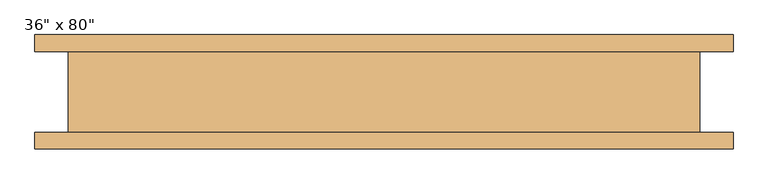
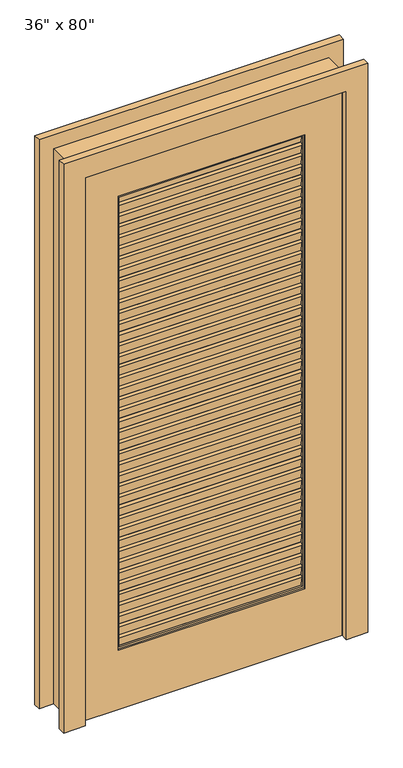
"""IFC4 building model written with IfcOpenShell, lengths in millimetres: door geometry."""

import ifcopenshell
import ifcopenshell.guid

model = None  # the IFC model being written
_history = None  # IfcOwnerHistory: only IFC2X3 demands one
_inside = {}  # id of a spatial element -> (the spatial element, [elements in it])
_under = {}  # id of a project, library or spatial element -> (it, [spatial elements below it])
_declared = {}  # id of a project -> (the project, [libraries it declares])
_typed = {}  # id of a type object -> (the type object, [elements of that type])
_made_of = {}  # id of a material, layer set ... -> (it, [elements and type objects made of it])


def new_model(schema):
    """Start an empty IFC model of exactly this schema.

    Asked for "IFC4X3", IfcOpenShell would pick the latest addendum, in which some entities
    have other attributes; the version numbers below select the first issue.
    IFC2X3 requires an IfcOwnerHistory on every rooted entity: one is made here for all.
    """
    global model, _history
    if schema == "IFC4X3":
        model = ifcopenshell.file(schema_version=(4, 3, 0, 0))
    else:
        model = ifcopenshell.file(schema=schema)
    _inside.clear()
    _under.clear()
    _declared.clear()
    _typed.clear()
    _made_of.clear()
    _history = None
    if model.schema == "IFC2X3":
        org = make("IfcOrganization", Name="unknown")
        user = make(
            "IfcPersonAndOrganization",
            ThePerson=make("IfcPerson", FamilyName="unknown"),
            TheOrganization=org,
        )
        app = make(
            "IfcApplication",
            ApplicationDeveloper=org,
            Version="unknown",
            ApplicationFullName="unknown",
            ApplicationIdentifier="unknown",
        )
        _history = make(
            "IfcOwnerHistory",
            OwningUser=user,
            OwningApplication=app,
            ChangeAction="ADDED",
            CreationDate=0,
        )
    return model


def make(cls, **values):
    """One entity of the class cls with the attributes given. An attribute that is None is left unset."""
    return model.create_entity(
        cls, **{name: value for name, value in values.items() if value is not None}
    )


def rooted(cls, **values):
    """An entity with a GlobalId (a new one), such as an element, a storey or a relation."""
    return make(cls, GlobalId=ifcopenshell.guid.new(), OwnerHistory=_history, **values)


def si_unit(unit_type, name, prefix=None):
    """IfcSIUnit, for example si_unit("LENGTHUNIT", "METRE", prefix="MILLI")."""
    return make("IfcSIUnit", UnitType=unit_type, Prefix=prefix, Name=name)


def assignment(units):
    """IfcUnitAssignment: the units of a project."""
    return None if units is None else make("IfcUnitAssignment", Units=units)


def point(xyz):
    """IfcCartesianPoint."""
    return None if xyz is None else make("IfcCartesianPoint", Coordinates=xyz)


def direction(xyz):
    """IfcDirection."""
    return None if xyz is None else make("IfcDirection", DirectionRatios=xyz)


def frame(location, z_axis=None, x_axis=None):
    """IfcAxis2Placement3D, a coordinate frame: its origin and axes. An axis left out is left unset."""
    return make(
        "IfcAxis2Placement3D",
        Location=point(location),
        Axis=direction(z_axis),
        RefDirection=direction(x_axis),
    )


def frame_2d(location, x_axis=None):
    """IfcAxis2Placement2D, a coordinate frame in the plane: its origin and x axis."""
    return make(
        "IfcAxis2Placement2D", Location=point(location), RefDirection=direction(x_axis)
    )


def origin():
    """The frame at (0, 0, 0) with its axes left unset."""
    return frame((0.0, 0.0, 0.0))


def place(relative_to, where):
    """IfcLocalPlacement: puts the frame where relative to a parent placement (None: the world)."""
    return make(
        "IfcLocalPlacement", PlacementRelTo=relative_to, RelativePlacement=where
    )


def context(
    kind, dimensions, precision=None, world=None, true_north=None, identifier=None
):
    """IfcGeometricRepresentationContext, for example the 3D "Model" context."""
    return make(
        "IfcGeometricRepresentationContext",
        ContextIdentifier=identifier,
        ContextType=kind,
        CoordinateSpaceDimension=dimensions,
        Precision=precision,
        WorldCoordinateSystem=world,
        TrueNorth=true_north,
    )


def project(units=None, contexts=None):
    """IfcProject with its units and contexts."""
    return rooted(
        "IfcProject",
        Name="project",
        RepresentationContexts=contexts,
        UnitsInContext=assignment(units),
    )


def spatial(cls, under=None, at=None, **own):
    """A site, building, storey or space (cls), placed at a placement, below another one or the project."""
    s = rooted(cls, ObjectPlacement=at, **own)
    if under is not None:
        _under.setdefault(under.id(), (under, []))[1].append(s)
    return s


def polyline(points):
    """IfcPolyline through the points."""
    return make("IfcPolyline", Points=[point(p) for p in points])


def circle_curve(where, radius):
    """IfcCircle in the frame where."""
    return make("IfcCircle", Position=where, Radius=radius)


def trimmed(basis, trim1, trim2, sense, master):
    """IfcTrimmedCurve: the piece of a basis curve between two trims."""
    return make(
        "IfcTrimmedCurve",
        BasisCurve=basis,
        Trim1=trim1,
        Trim2=trim2,
        SenseAgreement=sense,
        MasterRepresentation=master,
    )


def segment(curve, same_sense, transition):
    """IfcCompositeCurveSegment."""
    return make(
        "IfcCompositeCurveSegment",
        Transition=transition,
        SameSense=same_sense,
        ParentCurve=curve,
    )


def composite_curve(segments, self_intersect=None):
    """IfcCompositeCurve: segments joined end to end."""
    return make("IfcCompositeCurve", Segments=segments, SelfIntersect=self_intersect)


def outline(outer, holes=None, kind="AREA"):
    """IfcArbitraryClosedProfileDef: a profile drawn as a closed curve; with holes, ...WithVoids."""
    if holes is None:
        return make("IfcArbitraryClosedProfileDef", ProfileType=kind, OuterCurve=outer)
    return make(
        "IfcArbitraryProfileDefWithVoids",
        ProfileType=kind,
        OuterCurve=outer,
        InnerCurves=holes,
    )


def extrude(swept, where, along, depth):
    """IfcExtrudedAreaSolid: the profile swept, set in the frame where, extruded along a direction by depth."""
    return make(
        "IfcExtrudedAreaSolid",
        SweptArea=swept,
        Position=where,
        ExtrudedDirection=direction(along),
        Depth=depth,
    )


def faces_of(points, faces, orient=None, outer=None):
    """IfcFace entities. A face is a list of loops; a loop is a list of indices into points, from 0.

    orient and outer hold one flag for each loop. By default every Orientation is true, the
    first loop of a face is its IfcFaceOuterBound and the others are IfcFaceBound.
    """
    made = []
    for i, loops in enumerate(faces):
        bounds = []
        for j, loop in enumerate(loops):
            is_outer = j == 0 if outer is None else outer[i][j]
            bounds.append(
                make(
                    "IfcFaceOuterBound" if is_outer else "IfcFaceBound",
                    Bound=make("IfcPolyLoop", Polygon=[points[k] for k in loop]),
                    Orientation=True if orient is None else orient[i][j],
                )
            )
        made.append(make("IfcFace", Bounds=bounds))
    return made


def faceted_brep(points, faces, orient=None, outer=None, voids=None):
    """IfcFacetedBrep: a solid bounded by flat faces; with voids (closed shells), ...WithVoids."""
    shared = [point(p) for p in points]
    hull = make("IfcClosedShell", CfsFaces=faces_of(shared, faces, orient, outer))
    if voids is None:
        return make("IfcFacetedBrep", Outer=hull)
    return make(
        "IfcFacetedBrepWithVoids",
        Outer=hull,
        Voids=[
            make(cls, CfsFaces=faces_of(shared, fs, o, b)) for cls, fs, o, b in voids
        ],
    )


def shape(context_of_items, identifier, shape_type, items):
    """IfcShapeRepresentation: the items that make up one representation, for example the "Body"."""
    return make(
        "IfcShapeRepresentation",
        ContextOfItems=context_of_items,
        RepresentationIdentifier=identifier,
        RepresentationType=shape_type,
        Items=items,
    )


def source(mapping_origin, context_of_items, identifier, shape_type, items):
    """IfcRepresentationMap: a shape defined once, which mapped items show again and again."""
    return make(
        "IfcRepresentationMap",
        MappingOrigin=mapping_origin,
        MappedRepresentation=shape(context_of_items, identifier, shape_type, items),
    )


def transform(
    local_origin,
    x_axis=None,
    y_axis=None,
    z_axis=None,
    scale=None,
    scale2=None,
    scale3=None,
    uniform=True,
):
    """IfcCartesianTransformationOperator3D, or its non-uniform kind. x_axis, y_axis, z_axis: its Axis1, 2, 3."""
    if uniform:
        return make(
            "IfcCartesianTransformationOperator3D",
            Axis1=direction(x_axis),
            Axis2=direction(y_axis),
            LocalOrigin=point(local_origin),
            Scale=scale,
            Axis3=direction(z_axis),
        )
    return make(
        "IfcCartesianTransformationOperator3DnonUniform",
        Axis1=direction(x_axis),
        Axis2=direction(y_axis),
        LocalOrigin=point(local_origin),
        Scale=scale,
        Axis3=direction(z_axis),
        Scale2=scale2,
        Scale3=scale3,
    )


def mapped(mapping_source, mapping_target):
    """IfcMappedItem: shows the shape of a source again, moved by a transform."""
    return make(
        "IfcMappedItem", MappingSource=mapping_source, MappingTarget=mapping_target
    )


def made_of(thing, what):
    """Note that an element or type object is made of a material, layer set ...; save() writes the relation."""
    if what is not None:
        _made_of.setdefault(what.id(), (what, []))[1].append(thing)
    return thing


def element(
    cls,
    number,
    at=None,
    inside=None,
    cuts=None,
    type_object=None,
    material=None,
    context=None,
    identifier="Body",
    shape_type=None,
    held_by="IfcProductDefinitionShape",
    body=None,
    shapes=None,
    **own,
):
    """One element of the class cls, such as IfcWall. Its Tag is "e" and its number.

    at: its placement. inside: the storey or other place that contains it. cuts: it is an
    opening in that element (IfcRelVoidsElement). A single representation is given by context,
    identifier, shape_type and body (its items); several are given by shapes. held_by: the class
    of the entity that holds the representations. save() writes the other relations.
    """
    e = rooted(cls, Tag="e%d" % number, ObjectPlacement=at, **own)
    if body is not None:
        shapes = [shape(context, identifier, shape_type, body)]
    if shapes is not None:
        e.Representation = make(held_by, Representations=shapes)
    if inside is not None:
        _inside.setdefault(inside.id(), (inside, []))[1].append(e)
    if cuts is not None:
        rooted(
            "IfcRelVoidsElement", RelatingBuildingElement=cuts, RelatedOpeningElement=e
        )
    if type_object is not None:
        _typed.setdefault(type_object.id(), (type_object, []))[1].append(e)
    return made_of(e, material)


def aggregate(whole, parts):
    """IfcRelAggregates: a whole, such as a stair, and the parts it consists of."""
    return rooted("IfcRelAggregates", RelatingObject=whole, RelatedObjects=parts)


def save(model, path):
    """Write the relations noted so far, then the file.

    IfcRelAggregates (storeys below a building ...), IfcRelContainedInSpatialStructure (elements
    in a storey), IfcRelDefinesByType, IfcRelAssociatesMaterial and IfcRelDeclares: one each for
    every whole, place, type object, material and project.
    """
    for whole, parts in _under.values():
        aggregate(whole, parts)
    for where, things in _inside.values():
        rooted(
            "IfcRelContainedInSpatialStructure",
            RelatedElements=things,
            RelatingStructure=where,
        )
    for kind, things in _typed.values():
        rooted("IfcRelDefinesByType", RelatedObjects=things, RelatingType=kind)
    for what, things in _made_of.values():
        rooted("IfcRelAssociatesMaterial", RelatedObjects=things, RelatingMaterial=what)
    for by, libraries in _declared.values():
        rooted("IfcRelDeclares", RelatingContext=by, RelatedDefinitions=libraries)
    model.write(path)


def door_294ae2c4(model_context):
    return source(origin(), model_context, "Body", "SolidModel", [
        extrude(outline(composite_curve([segment(polyline([(-25.516257, 1899.8217262), (-31.75, 1867.3157738), (-31.75, 1857.7907738), (-47.625, 1857.7907738), (-47.625, 1867.3157738), (-53.858743, 1899.8217262)]), True, "CONTINUOUS"), segment(trimmed(circle_curve(frame_2d((-47.625, 1901.03125)), 6.35), [point((-53.858743, 1899.8217262))], [point((-47.625, 1907.38125))], False, "CARTESIAN"), True, "CONTINUOUS"), segment(polyline([(-47.625, 1907.38125), (-47.625, 1899.44375), (-31.75, 1899.44375), (-31.75, 1907.38125)]), True, "CONTINUOUS"), segment(trimmed(circle_curve(frame_2d((-31.75, 1901.03125)), 6.35), [point((-31.75, 1907.38125))], [point((-25.516257, 1899.8217262))], False, "CARTESIAN"), True, "CONTINUOUS")], self_intersect=False)), frame((-327.025, 0.0, 0.0), z_axis=(1.0, 0.0, 0.0), x_axis=(0.0, 1.0, 0.0)), (0.0, 0.0, 1.0), 654.05),
        extrude(outline(composite_curve([segment(polyline([(-25.516257, 1859.75625), (-31.75, 1827.2502976), (-31.75, 1817.7252976), (-47.625, 1817.7252976), (-47.625, 1827.2502976), (-53.858743, 1859.75625)]), True, "CONTINUOUS"), segment(trimmed(circle_curve(frame_2d((-47.625, 1860.9657738)), 6.35), [point((-53.858743, 1859.75625))], [point((-47.625, 1867.3157738))], False, "CARTESIAN"), True, "CONTINUOUS"), segment(polyline([(-47.625, 1867.3157738), (-47.625, 1859.3782738), (-31.75, 1859.3782738), (-31.75, 1867.3157738)]), True, "CONTINUOUS"), segment(trimmed(circle_curve(frame_2d((-31.75, 1860.9657738)), 6.35), [point((-31.75, 1867.3157738))], [point((-25.516257, 1859.75625))], False, "CARTESIAN"), True, "CONTINUOUS")], self_intersect=False)), frame((-327.025, 0.0, 0.0), z_axis=(1.0, 0.0, 0.0), x_axis=(0.0, 1.0, 0.0)), (0.0, 0.0, 1.0), 654.05),
        extrude(outline(composite_curve([segment(polyline([(-25.516257, 1819.6907738), (-31.75, 1787.1848214), (-31.75, 1777.6598214), (-47.625, 1777.6598214), (-47.625, 1787.1848214), (-53.858743, 1819.6907738)]), True, "CONTINUOUS"), segment(trimmed(circle_curve(frame_2d((-47.625, 1820.9002976)), 6.35), [point((-53.858743, 1819.6907738))], [point((-47.625, 1827.2502976))], False, "CARTESIAN"), True, "CONTINUOUS"), segment(polyline([(-47.625, 1827.2502976), (-47.625, 1819.3127976), (-31.75, 1819.3127976), (-31.75, 1827.2502976)]), True, "CONTINUOUS"), segment(trimmed(circle_curve(frame_2d((-31.75, 1820.9002976)), 6.35), [point((-31.75, 1827.2502976))], [point((-25.516257, 1819.6907738))], False, "CARTESIAN"), True, "CONTINUOUS")], self_intersect=False)), frame((-327.025, 0.0, 0.0), z_axis=(1.0, 0.0, 0.0), x_axis=(0.0, 1.0, 0.0)), (0.0, 0.0, 1.0), 654.05),
        extrude(outline(composite_curve([segment(polyline([(-25.516257, 1779.6252976), (-31.75, 1747.1193452), (-31.75, 1737.5943452), (-47.625, 1737.5943452), (-47.625, 1747.1193452), (-53.858743, 1779.6252976)]), True, "CONTINUOUS"), segment(trimmed(circle_curve(frame_2d((-47.625, 1780.8348214)), 6.35), [point((-53.858743, 1779.6252976))], [point((-47.625, 1787.1848214))], False, "CARTESIAN"), True, "CONTINUOUS"), segment(polyline([(-47.625, 1787.1848214), (-47.625, 1779.2473214), (-31.75, 1779.2473214), (-31.75, 1787.1848214)]), True, "CONTINUOUS"), segment(trimmed(circle_curve(frame_2d((-31.75, 1780.8348214)), 6.35), [point((-31.75, 1787.1848214))], [point((-25.516257, 1779.6252976))], False, "CARTESIAN"), True, "CONTINUOUS")], self_intersect=False)), frame((-327.025, 0.0, 0.0), z_axis=(1.0, 0.0, 0.0), x_axis=(0.0, 1.0, 0.0)), (0.0, 0.0, 1.0), 654.05),
        extrude(outline(composite_curve([segment(polyline([(-25.516257, 1739.5598214), (-31.75, 1707.053869), (-31.75, 1697.528869), (-47.625, 1697.528869), (-47.625, 1707.053869), (-53.858743, 1739.5598214)]), True, "CONTINUOUS"), segment(trimmed(circle_curve(frame_2d((-47.625, 1740.7693452)), 6.35), [point((-53.858743, 1739.5598214))], [point((-47.625, 1747.1193452))], False, "CARTESIAN"), True, "CONTINUOUS"), segment(polyline([(-47.625, 1747.1193452), (-47.625, 1739.1818452), (-31.75, 1739.1818452), (-31.75, 1747.1193452)]), True, "CONTINUOUS"), segment(trimmed(circle_curve(frame_2d((-31.75, 1740.7693452)), 6.35), [point((-31.75, 1747.1193452))], [point((-25.516257, 1739.5598214))], False, "CARTESIAN"), True, "CONTINUOUS")], self_intersect=False)), frame((-327.025, 0.0, 0.0), z_axis=(1.0, 0.0, 0.0), x_axis=(0.0, 1.0, 0.0)), (0.0, 0.0, 1.0), 654.05),
        extrude(outline(composite_curve([segment(polyline([(-25.516257, 1699.4943452), (-31.75, 1666.9883929), (-31.75, 1657.4633929), (-47.625, 1657.4633929), (-47.625, 1666.9883929), (-53.858743, 1699.4943452)]), True, "CONTINUOUS"), segment(trimmed(circle_curve(frame_2d((-47.625, 1700.703869)), 6.35), [point((-53.858743, 1699.4943452))], [point((-47.625, 1707.053869))], False, "CARTESIAN"), True, "CONTINUOUS"), segment(polyline([(-47.625, 1707.053869), (-47.625, 1699.116369), (-31.75, 1699.116369), (-31.75, 1707.053869)]), True, "CONTINUOUS"), segment(trimmed(circle_curve(frame_2d((-31.75, 1700.703869)), 6.35), [point((-31.75, 1707.053869))], [point((-25.516257, 1699.4943452))], False, "CARTESIAN"), True, "CONTINUOUS")], self_intersect=False)), frame((-327.025, 0.0, 0.0), z_axis=(1.0, 0.0, 0.0), x_axis=(0.0, 1.0, 0.0)), (0.0, 0.0, 1.0), 654.05),
        extrude(outline(composite_curve([segment(polyline([(-25.516257, 1659.428869), (-31.75, 1626.9229167), (-31.75, 1617.3979167), (-47.625, 1617.3979167), (-47.625, 1626.9229167), (-53.858743, 1659.428869)]), True, "CONTINUOUS"), segment(trimmed(circle_curve(frame_2d((-47.625, 1660.6383929)), 6.35), [point((-53.858743, 1659.428869))], [point((-47.625, 1666.9883929))], False, "CARTESIAN"), True, "CONTINUOUS"), segment(polyline([(-47.625, 1666.9883929), (-47.625, 1659.0508929), (-31.75, 1659.0508929), (-31.75, 1666.9883929)]), True, "CONTINUOUS"), segment(trimmed(circle_curve(frame_2d((-31.75, 1660.6383929)), 6.35), [point((-31.75, 1666.9883929))], [point((-25.516257, 1659.428869))], False, "CARTESIAN"), True, "CONTINUOUS")], self_intersect=False)), frame((-327.025, 0.0, 0.0), z_axis=(1.0, 0.0, 0.0), x_axis=(0.0, 1.0, 0.0)), (0.0, 0.0, 1.0), 654.05),
        extrude(outline(composite_curve([segment(polyline([(-25.516257, 1619.3633929), (-31.75, 1586.8574405), (-31.75, 1577.3324405), (-47.625, 1577.3324405), (-47.625, 1586.8574405), (-53.858743, 1619.3633929)]), True, "CONTINUOUS"), segment(trimmed(circle_curve(frame_2d((-47.625, 1620.5729167)), 6.35), [point((-53.858743, 1619.3633929))], [point((-47.625, 1626.9229167))], False, "CARTESIAN"), True, "CONTINUOUS"), segment(polyline([(-47.625, 1626.9229167), (-47.625, 1618.9854167), (-31.75, 1618.9854167), (-31.75, 1626.9229167)]), True, "CONTINUOUS"), segment(trimmed(circle_curve(frame_2d((-31.75, 1620.5729167)), 6.35), [point((-31.75, 1626.9229167))], [point((-25.516257, 1619.3633929))], False, "CARTESIAN"), True, "CONTINUOUS")], self_intersect=False)), frame((-327.025, 0.0, 0.0), z_axis=(1.0, 0.0, 0.0), x_axis=(0.0, 1.0, 0.0)), (0.0, 0.0, 1.0), 654.05),
        extrude(outline(composite_curve([segment(polyline([(-25.516257, 1579.2979167), (-31.75, 1546.7919643), (-31.75, 1537.2669643), (-47.625, 1537.2669643), (-47.625, 1546.7919643), (-53.858743, 1579.2979167)]), True, "CONTINUOUS"), segment(trimmed(circle_curve(frame_2d((-47.625, 1580.5074405)), 6.35), [point((-53.858743, 1579.2979167))], [point((-47.625, 1586.8574405))], False, "CARTESIAN"), True, "CONTINUOUS"), segment(polyline([(-47.625, 1586.8574405), (-47.625, 1578.9199405), (-31.75, 1578.9199405), (-31.75, 1586.8574405)]), True, "CONTINUOUS"), segment(trimmed(circle_curve(frame_2d((-31.75, 1580.5074405)), 6.35), [point((-31.75, 1586.8574405))], [point((-25.516257, 1579.2979167))], False, "CARTESIAN"), True, "CONTINUOUS")], self_intersect=False)), frame((-327.025, 0.0, 0.0), z_axis=(1.0, 0.0, 0.0), x_axis=(0.0, 1.0, 0.0)), (0.0, 0.0, 1.0), 654.05),
        extrude(outline(composite_curve([segment(polyline([(-25.516257, 1539.2324405), (-31.75, 1506.7264881), (-31.75, 1497.2014881), (-47.625, 1497.2014881), (-47.625, 1506.7264881), (-53.858743, 1539.2324405)]), True, "CONTINUOUS"), segment(trimmed(circle_curve(frame_2d((-47.625, 1540.4419643)), 6.35), [point((-53.858743, 1539.2324405))], [point((-47.625, 1546.7919643))], False, "CARTESIAN"), True, "CONTINUOUS"), segment(polyline([(-47.625, 1546.7919643), (-47.625, 1538.8544643), (-31.75, 1538.8544643), (-31.75, 1546.7919643)]), True, "CONTINUOUS"), segment(trimmed(circle_curve(frame_2d((-31.75, 1540.4419643)), 6.35), [point((-31.75, 1546.7919643))], [point((-25.516257, 1539.2324405))], False, "CARTESIAN"), True, "CONTINUOUS")], self_intersect=False)), frame((-327.025, 0.0, 0.0), z_axis=(1.0, 0.0, 0.0), x_axis=(0.0, 1.0, 0.0)), (0.0, 0.0, 1.0), 654.05),
        extrude(outline(composite_curve([segment(polyline([(-25.516257, 1499.1669643), (-31.75, 1466.6610119), (-31.75, 1457.1360119), (-47.625, 1457.1360119), (-47.625, 1466.6610119), (-53.858743, 1499.1669643)]), True, "CONTINUOUS"), segment(trimmed(circle_curve(frame_2d((-47.625, 1500.3764881)), 6.35), [point((-53.858743, 1499.1669643))], [point((-47.625, 1506.7264881))], False, "CARTESIAN"), True, "CONTINUOUS"), segment(polyline([(-47.625, 1506.7264881), (-47.625, 1498.7889881), (-31.75, 1498.7889881), (-31.75, 1506.7264881)]), True, "CONTINUOUS"), segment(trimmed(circle_curve(frame_2d((-31.75, 1500.3764881)), 6.35), [point((-31.75, 1506.7264881))], [point((-25.516257, 1499.1669643))], False, "CARTESIAN"), True, "CONTINUOUS")], self_intersect=False)), frame((-327.025, 0.0, 0.0), z_axis=(1.0, 0.0, 0.0), x_axis=(0.0, 1.0, 0.0)), (0.0, 0.0, 1.0), 654.05),
        extrude(outline(composite_curve([segment(polyline([(-25.516257, 1459.1014881), (-31.75, 1426.5955357), (-31.75, 1417.0705357), (-47.625, 1417.0705357), (-47.625, 1426.5955357), (-53.858743, 1459.1014881)]), True, "CONTINUOUS"), segment(trimmed(circle_curve(frame_2d((-47.625, 1460.3110119)), 6.35), [point((-53.858743, 1459.1014881))], [point((-47.625, 1466.6610119))], False, "CARTESIAN"), True, "CONTINUOUS"), segment(polyline([(-47.625, 1466.6610119), (-47.625, 1458.7235119), (-31.75, 1458.7235119), (-31.75, 1466.6610119)]), True, "CONTINUOUS"), segment(trimmed(circle_curve(frame_2d((-31.75, 1460.3110119)), 6.35), [point((-31.75, 1466.6610119))], [point((-25.516257, 1459.1014881))], False, "CARTESIAN"), True, "CONTINUOUS")], self_intersect=False)), frame((-327.025, 0.0, 0.0), z_axis=(1.0, 0.0, 0.0), x_axis=(0.0, 1.0, 0.0)), (0.0, 0.0, 1.0), 654.05),
        extrude(outline(composite_curve([segment(polyline([(-25.516257, 1419.0360119), (-31.75, 1386.5300595), (-31.75, 1377.0050595), (-47.625, 1377.0050595), (-47.625, 1386.5300595), (-53.858743, 1419.0360119)]), True, "CONTINUOUS"), segment(trimmed(circle_curve(frame_2d((-47.625, 1420.2455357)), 6.35), [point((-53.858743, 1419.0360119))], [point((-47.625, 1426.5955357))], False, "CARTESIAN"), True, "CONTINUOUS"), segment(polyline([(-47.625, 1426.5955357), (-47.625, 1418.6580357), (-31.75, 1418.6580357), (-31.75, 1426.5955357)]), True, "CONTINUOUS"), segment(trimmed(circle_curve(frame_2d((-31.75, 1420.2455357)), 6.35), [point((-31.75, 1426.5955357))], [point((-25.516257, 1419.0360119))], False, "CARTESIAN"), True, "CONTINUOUS")], self_intersect=False)), frame((-327.025, 0.0, 0.0), z_axis=(1.0, 0.0, 0.0), x_axis=(0.0, 1.0, 0.0)), (0.0, 0.0, 1.0), 654.05),
        extrude(outline(composite_curve([segment(polyline([(-25.516257, 1378.9705357), (-31.75, 1346.4645833), (-31.75, 1336.9395833), (-47.625, 1336.9395833), (-47.625, 1346.4645833), (-53.858743, 1378.9705357)]), True, "CONTINUOUS"), segment(trimmed(circle_curve(frame_2d((-47.625, 1380.1800595)), 6.35), [point((-53.858743, 1378.9705357))], [point((-47.625, 1386.5300595))], False, "CARTESIAN"), True, "CONTINUOUS"), segment(polyline([(-47.625, 1386.5300595), (-47.625, 1378.5925595), (-31.75, 1378.5925595), (-31.75, 1386.5300595)]), True, "CONTINUOUS"), segment(trimmed(circle_curve(frame_2d((-31.75, 1380.1800595)), 6.35), [point((-31.75, 1386.5300595))], [point((-25.516257, 1378.9705357))], False, "CARTESIAN"), True, "CONTINUOUS")], self_intersect=False)), frame((-327.025, 0.0, 0.0), z_axis=(1.0, 0.0, 0.0), x_axis=(0.0, 1.0, 0.0)), (0.0, 0.0, 1.0), 654.05),
        extrude(outline(composite_curve([segment(polyline([(-25.516257, 1338.9050595), (-31.75, 1306.3991071), (-31.75, 1296.8741071), (-47.625, 1296.8741071), (-47.625, 1306.3991071), (-53.858743, 1338.9050595)]), True, "CONTINUOUS"), segment(trimmed(circle_curve(frame_2d((-47.625, 1340.1145833)), 6.35), [point((-53.858743, 1338.9050595))], [point((-47.625, 1346.4645833))], False, "CARTESIAN"), True, "CONTINUOUS"), segment(polyline([(-47.625, 1346.4645833), (-47.625, 1338.5270833), (-31.75, 1338.5270833), (-31.75, 1346.4645833)]), True, "CONTINUOUS"), segment(trimmed(circle_curve(frame_2d((-31.75, 1340.1145833)), 6.35), [point((-31.75, 1346.4645833))], [point((-25.516257, 1338.9050595))], False, "CARTESIAN"), True, "CONTINUOUS")], self_intersect=False)), frame((-327.025, 0.0, 0.0), z_axis=(1.0, 0.0, 0.0), x_axis=(0.0, 1.0, 0.0)), (0.0, 0.0, 1.0), 654.05),
        extrude(outline(composite_curve([segment(polyline([(-25.516257, 1298.8395833), (-31.75, 1266.333631), (-31.75, 1256.808631), (-47.625, 1256.808631), (-47.625, 1266.333631), (-53.858743, 1298.8395833)]), True, "CONTINUOUS"), segment(trimmed(circle_curve(frame_2d((-47.625, 1300.0491071)), 6.35), [point((-53.858743, 1298.8395833))], [point((-47.625, 1306.3991071))], False, "CARTESIAN"), True, "CONTINUOUS"), segment(polyline([(-47.625, 1306.3991071), (-47.625, 1298.4616071), (-31.75, 1298.4616071), (-31.75, 1306.3991071)]), True, "CONTINUOUS"), segment(trimmed(circle_curve(frame_2d((-31.75, 1300.0491071)), 6.35), [point((-31.75, 1306.3991071))], [point((-25.516257, 1298.8395833))], False, "CARTESIAN"), True, "CONTINUOUS")], self_intersect=False)), frame((-327.025, 0.0, 0.0), z_axis=(1.0, 0.0, 0.0), x_axis=(0.0, 1.0, 0.0)), (0.0, 0.0, 1.0), 654.05),
        extrude(outline(composite_curve([segment(polyline([(-25.516257, 1258.7741071), (-31.75, 1226.2681548), (-31.75, 1216.7431548), (-47.625, 1216.7431548), (-47.625, 1226.2681548), (-53.858743, 1258.7741071)]), True, "CONTINUOUS"), segment(trimmed(circle_curve(frame_2d((-47.625, 1259.983631)), 6.35), [point((-53.858743, 1258.7741071))], [point((-47.625, 1266.333631))], False, "CARTESIAN"), True, "CONTINUOUS"), segment(polyline([(-47.625, 1266.333631), (-47.625, 1258.396131), (-31.75, 1258.396131), (-31.75, 1266.333631)]), True, "CONTINUOUS"), segment(trimmed(circle_curve(frame_2d((-31.75, 1259.983631)), 6.35), [point((-31.75, 1266.333631))], [point((-25.516257, 1258.7741071))], False, "CARTESIAN"), True, "CONTINUOUS")], self_intersect=False)), frame((-327.025, 0.0, 0.0), z_axis=(1.0, 0.0, 0.0), x_axis=(0.0, 1.0, 0.0)), (0.0, 0.0, 1.0), 654.05),
        extrude(outline(composite_curve([segment(polyline([(-25.516257, 1218.708631), (-31.75, 1186.2026786), (-31.75, 1176.6776786), (-47.625, 1176.6776786), (-47.625, 1186.2026786), (-53.858743, 1218.708631)]), True, "CONTINUOUS"), segment(trimmed(circle_curve(frame_2d((-47.625, 1219.9181548)), 6.35), [point((-53.858743, 1218.708631))], [point((-47.625, 1226.2681548))], False, "CARTESIAN"), True, "CONTINUOUS"), segment(polyline([(-47.625, 1226.2681548), (-47.625, 1218.3306548), (-31.75, 1218.3306548), (-31.75, 1226.2681548)]), True, "CONTINUOUS"), segment(trimmed(circle_curve(frame_2d((-31.75, 1219.9181548)), 6.35), [point((-31.75, 1226.2681548))], [point((-25.516257, 1218.708631))], False, "CARTESIAN"), True, "CONTINUOUS")], self_intersect=False)), frame((-327.025, 0.0, 0.0), z_axis=(1.0, 0.0, 0.0), x_axis=(0.0, 1.0, 0.0)), (0.0, 0.0, 1.0), 654.05),
        extrude(outline(composite_curve([segment(polyline([(-25.516257, 1178.6431548), (-31.75, 1146.1372024), (-31.75, 1136.6122024), (-47.625, 1136.6122024), (-47.625, 1146.1372024), (-53.858743, 1178.6431548)]), True, "CONTINUOUS"), segment(trimmed(circle_curve(frame_2d((-47.625, 1179.8526786)), 6.35), [point((-53.858743, 1178.6431548))], [point((-47.625, 1186.2026786))], False, "CARTESIAN"), True, "CONTINUOUS"), segment(polyline([(-47.625, 1186.2026786), (-47.625, 1178.2651786), (-31.75, 1178.2651786), (-31.75, 1186.2026786)]), True, "CONTINUOUS"), segment(trimmed(circle_curve(frame_2d((-31.75, 1179.8526786)), 6.35), [point((-31.75, 1186.2026786))], [point((-25.516257, 1178.6431548))], False, "CARTESIAN"), True, "CONTINUOUS")], self_intersect=False)), frame((-327.025, 0.0, 0.0), z_axis=(1.0, 0.0, 0.0), x_axis=(0.0, 1.0, 0.0)), (0.0, 0.0, 1.0), 654.05),
        extrude(outline(composite_curve([segment(polyline([(-25.516257, 1138.5776786), (-31.75, 1106.0717262), (-31.75, 1096.5467262), (-47.625, 1096.5467262), (-47.625, 1106.0717262), (-53.858743, 1138.5776786)]), True, "CONTINUOUS"), segment(trimmed(circle_curve(frame_2d((-47.625, 1139.7872024)), 6.35), [point((-53.858743, 1138.5776786))], [point((-47.625, 1146.1372024))], False, "CARTESIAN"), True, "CONTINUOUS"), segment(polyline([(-47.625, 1146.1372024), (-47.625, 1138.1997024), (-31.75, 1138.1997024), (-31.75, 1146.1372024)]), True, "CONTINUOUS"), segment(trimmed(circle_curve(frame_2d((-31.75, 1139.7872024)), 6.35), [point((-31.75, 1146.1372024))], [point((-25.516257, 1138.5776786))], False, "CARTESIAN"), True, "CONTINUOUS")], self_intersect=False)), frame((-327.025, 0.0, 0.0), z_axis=(1.0, 0.0, 0.0), x_axis=(0.0, 1.0, 0.0)), (0.0, 0.0, 1.0), 654.05),
        extrude(outline(composite_curve([segment(polyline([(-25.516257, 1098.5122024), (-31.75, 1066.00625), (-31.75, 1056.48125), (-47.625, 1056.48125), (-47.625, 1066.00625), (-53.858743, 1098.5122024)]), True, "CONTINUOUS"), segment(trimmed(circle_curve(frame_2d((-47.625, 1099.7217262)), 6.35), [point((-53.858743, 1098.5122024))], [point((-47.625, 1106.0717262))], False, "CARTESIAN"), True, "CONTINUOUS"), segment(polyline([(-47.625, 1106.0717262), (-47.625, 1098.1342262), (-31.75, 1098.1342262), (-31.75, 1106.0717262)]), True, "CONTINUOUS"), segment(trimmed(circle_curve(frame_2d((-31.75, 1099.7217262)), 6.35), [point((-31.75, 1106.0717262))], [point((-25.516257, 1098.5122024))], False, "CARTESIAN"), True, "CONTINUOUS")], self_intersect=False)), frame((-327.025, 0.0, 0.0), z_axis=(1.0, 0.0, 0.0), x_axis=(0.0, 1.0, 0.0)), (0.0, 0.0, 1.0), 654.05),
        extrude(outline(composite_curve([segment(polyline([(-25.516257, 1058.4467262), (-31.75, 1025.9407738), (-31.75, 1016.4157738), (-47.625, 1016.4157738), (-47.625, 1025.9407738), (-53.858743, 1058.4467262)]), True, "CONTINUOUS"), segment(trimmed(circle_curve(frame_2d((-47.625, 1059.65625)), 6.35), [point((-53.858743, 1058.4467262))], [point((-47.625, 1066.00625))], False, "CARTESIAN"), True, "CONTINUOUS"), segment(polyline([(-47.625, 1066.00625), (-47.625, 1058.06875), (-31.75, 1058.06875), (-31.75, 1066.00625)]), True, "CONTINUOUS"), segment(trimmed(circle_curve(frame_2d((-31.75, 1059.65625)), 6.35), [point((-31.75, 1066.00625))], [point((-25.516257, 1058.4467262))], False, "CARTESIAN"), True, "CONTINUOUS")], self_intersect=False)), frame((-327.025, 0.0, 0.0), z_axis=(1.0, 0.0, 0.0), x_axis=(0.0, 1.0, 0.0)), (0.0, 0.0, 1.0), 654.05),
        extrude(outline(composite_curve([segment(polyline([(-25.516257, 1018.38125), (-31.75, 985.8752976), (-31.75, 976.3502976), (-47.625, 976.3502976), (-47.625, 985.8752976), (-53.858743, 1018.38125)]), True, "CONTINUOUS"), segment(trimmed(circle_curve(frame_2d((-47.625, 1019.5907738)), 6.35), [point((-53.858743, 1018.38125))], [point((-47.625, 1025.9407738))], False, "CARTESIAN"), True, "CONTINUOUS"), segment(polyline([(-47.625, 1025.9407738), (-47.625, 1018.0032738), (-31.75, 1018.0032738), (-31.75, 1025.9407738)]), True, "CONTINUOUS"), segment(trimmed(circle_curve(frame_2d((-31.75, 1019.5907738)), 6.35), [point((-31.75, 1025.9407738))], [point((-25.516257, 1018.38125))], False, "CARTESIAN"), True, "CONTINUOUS")], self_intersect=False)), frame((-327.025, 0.0, 0.0), z_axis=(1.0, 0.0, 0.0), x_axis=(0.0, 1.0, 0.0)), (0.0, 0.0, 1.0), 654.05),
        extrude(outline(composite_curve([segment(polyline([(-25.516257, 978.3157738), (-31.75, 945.8098214), (-31.75, 936.2848214), (-47.625, 936.2848214), (-47.625, 945.8098214), (-53.858743, 978.3157738)]), True, "CONTINUOUS"), segment(trimmed(circle_curve(frame_2d((-47.625, 979.5252976)), 6.35), [point((-53.858743, 978.3157738))], [point((-47.625, 985.8752976))], False, "CARTESIAN"), True, "CONTINUOUS"), segment(polyline([(-47.625, 985.8752976), (-47.625, 977.9377976), (-31.75, 977.9377976), (-31.75, 985.8752976)]), True, "CONTINUOUS"), segment(trimmed(circle_curve(frame_2d((-31.75, 979.5252976)), 6.35), [point((-31.75, 985.8752976))], [point((-25.516257, 978.3157738))], False, "CARTESIAN"), True, "CONTINUOUS")], self_intersect=False)), frame((-327.025, 0.0, 0.0), z_axis=(1.0, 0.0, 0.0), x_axis=(0.0, 1.0, 0.0)), (0.0, 0.0, 1.0), 654.05),
        extrude(outline(composite_curve([segment(polyline([(-25.516257, 938.2502976), (-31.75, 905.7443452), (-31.75, 896.2193452), (-47.625, 896.2193452), (-47.625, 905.7443452), (-53.858743, 938.2502976)]), True, "CONTINUOUS"), segment(trimmed(circle_curve(frame_2d((-47.625, 939.4598214)), 6.35), [point((-53.858743, 938.2502976))], [point((-47.625, 945.8098214))], False, "CARTESIAN"), True, "CONTINUOUS"), segment(polyline([(-47.625, 945.8098214), (-47.625, 937.8723214), (-31.75, 937.8723214), (-31.75, 945.8098214)]), True, "CONTINUOUS"), segment(trimmed(circle_curve(frame_2d((-31.75, 939.4598214)), 6.35), [point((-31.75, 945.8098214))], [point((-25.516257, 938.2502976))], False, "CARTESIAN"), True, "CONTINUOUS")], self_intersect=False)), frame((-327.025, 0.0, 0.0), z_axis=(1.0, 0.0, 0.0), x_axis=(0.0, 1.0, 0.0)), (0.0, 0.0, 1.0), 654.05),
        extrude(outline(composite_curve([segment(polyline([(-25.516257, 898.1848214), (-31.75, 865.678869), (-31.75, 856.153869), (-47.625, 856.153869), (-47.625, 865.678869), (-53.858743, 898.1848214)]), True, "CONTINUOUS"), segment(trimmed(circle_curve(frame_2d((-47.625, 899.3943452)), 6.35), [point((-53.858743, 898.1848214))], [point((-47.625, 905.7443452))], False, "CARTESIAN"), True, "CONTINUOUS"), segment(polyline([(-47.625, 905.7443452), (-47.625, 897.8068452), (-31.75, 897.8068452), (-31.75, 905.7443452)]), True, "CONTINUOUS"), segment(trimmed(circle_curve(frame_2d((-31.75, 899.3943452)), 6.35), [point((-31.75, 905.7443452))], [point((-25.516257, 898.1848214))], False, "CARTESIAN"), True, "CONTINUOUS")], self_intersect=False)), frame((-327.025, 0.0, 0.0), z_axis=(1.0, 0.0, 0.0), x_axis=(0.0, 1.0, 0.0)), (0.0, 0.0, 1.0), 654.05),
        extrude(outline(composite_curve([segment(polyline([(-25.516257, 858.1193452), (-31.75, 825.6133929), (-31.75, 816.0883929), (-47.625, 816.0883929), (-47.625, 825.6133929), (-53.858743, 858.1193452)]), True, "CONTINUOUS"), segment(trimmed(circle_curve(frame_2d((-47.625, 859.328869)), 6.35), [point((-53.858743, 858.1193452))], [point((-47.625, 865.678869))], False, "CARTESIAN"), True, "CONTINUOUS"), segment(polyline([(-47.625, 865.678869), (-47.625, 857.741369), (-31.75, 857.741369), (-31.75, 865.678869)]), True, "CONTINUOUS"), segment(trimmed(circle_curve(frame_2d((-31.75, 859.328869)), 6.35), [point((-31.75, 865.678869))], [point((-25.516257, 858.1193452))], False, "CARTESIAN"), True, "CONTINUOUS")], self_intersect=False)), frame((-327.025, 0.0, 0.0), z_axis=(1.0, 0.0, 0.0), x_axis=(0.0, 1.0, 0.0)), (0.0, 0.0, 1.0), 654.05),
        extrude(outline(composite_curve([segment(polyline([(-25.516257, 818.053869), (-31.75, 785.5479167), (-31.75, 776.0229167), (-47.625, 776.0229167), (-47.625, 785.5479167), (-53.858743, 818.053869)]), True, "CONTINUOUS"), segment(trimmed(circle_curve(frame_2d((-47.625, 819.2633929)), 6.35), [point((-53.858743, 818.053869))], [point((-47.625, 825.6133929))], False, "CARTESIAN"), True, "CONTINUOUS"), segment(polyline([(-47.625, 825.6133929), (-47.625, 817.6758929), (-31.75, 817.6758929), (-31.75, 825.6133929)]), True, "CONTINUOUS"), segment(trimmed(circle_curve(frame_2d((-31.75, 819.2633929)), 6.35), [point((-31.75, 825.6133929))], [point((-25.516257, 818.053869))], False, "CARTESIAN"), True, "CONTINUOUS")], self_intersect=False)), frame((-327.025, 0.0, 0.0), z_axis=(1.0, 0.0, 0.0), x_axis=(0.0, 1.0, 0.0)), (0.0, 0.0, 1.0), 654.05),
        extrude(outline(composite_curve([segment(polyline([(-25.516257, 777.9883929), (-31.75, 745.4824405), (-31.75, 735.9574405), (-47.625, 735.9574405), (-47.625, 745.4824405), (-53.858743, 777.9883929)]), True, "CONTINUOUS"), segment(trimmed(circle_curve(frame_2d((-47.625, 779.1979167)), 6.35), [point((-53.858743, 777.9883929))], [point((-47.625, 785.5479167))], False, "CARTESIAN"), True, "CONTINUOUS"), segment(polyline([(-47.625, 785.5479167), (-47.625, 777.6104167), (-31.75, 777.6104167), (-31.75, 785.5479167)]), True, "CONTINUOUS"), segment(trimmed(circle_curve(frame_2d((-31.75, 779.1979167)), 6.35), [point((-31.75, 785.5479167))], [point((-25.516257, 777.9883929))], False, "CARTESIAN"), True, "CONTINUOUS")], self_intersect=False)), frame((-327.025, 0.0, 0.0), z_axis=(1.0, 0.0, 0.0), x_axis=(0.0, 1.0, 0.0)), (0.0, 0.0, 1.0), 654.05),
        extrude(outline(composite_curve([segment(polyline([(-25.516257, 737.9229167), (-31.75, 705.4169643), (-31.75, 695.8919643), (-47.625, 695.8919643), (-47.625, 705.4169643), (-53.858743, 737.9229167)]), True, "CONTINUOUS"), segment(trimmed(circle_curve(frame_2d((-47.625, 739.1324405)), 6.35), [point((-53.858743, 737.9229167))], [point((-47.625, 745.4824405))], False, "CARTESIAN"), True, "CONTINUOUS"), segment(polyline([(-47.625, 745.4824405), (-47.625, 737.5449405), (-31.75, 737.5449405), (-31.75, 745.4824405)]), True, "CONTINUOUS"), segment(trimmed(circle_curve(frame_2d((-31.75, 739.1324405)), 6.35), [point((-31.75, 745.4824405))], [point((-25.516257, 737.9229167))], False, "CARTESIAN"), True, "CONTINUOUS")], self_intersect=False)), frame((-327.025, 0.0, 0.0), z_axis=(1.0, 0.0, 0.0), x_axis=(0.0, 1.0, 0.0)), (0.0, 0.0, 1.0), 654.05),
        extrude(outline(composite_curve([segment(polyline([(-25.516257, 697.8574405), (-31.75, 665.3514881), (-31.75, 655.8264881), (-47.625, 655.8264881), (-47.625, 665.3514881), (-53.858743, 697.8574405)]), True, "CONTINUOUS"), segment(trimmed(circle_curve(frame_2d((-47.625, 699.0669643)), 6.35), [point((-53.858743, 697.8574405))], [point((-47.625, 705.4169643))], False, "CARTESIAN"), True, "CONTINUOUS"), segment(polyline([(-47.625, 705.4169643), (-47.625, 697.4794643), (-31.75, 697.4794643), (-31.75, 705.4169643)]), True, "CONTINUOUS"), segment(trimmed(circle_curve(frame_2d((-31.75, 699.0669643)), 6.35), [point((-31.75, 705.4169643))], [point((-25.516257, 697.8574405))], False, "CARTESIAN"), True, "CONTINUOUS")], self_intersect=False)), frame((-327.025, 0.0, 0.0), z_axis=(1.0, 0.0, 0.0), x_axis=(0.0, 1.0, 0.0)), (0.0, 0.0, 1.0), 654.05),
        extrude(outline(composite_curve([segment(polyline([(-25.516257, 657.7919643), (-31.75, 625.2860119), (-31.75, 615.7610119), (-47.625, 615.7610119), (-47.625, 625.2860119), (-53.858743, 657.7919643)]), True, "CONTINUOUS"), segment(trimmed(circle_curve(frame_2d((-47.625, 659.0014881)), 6.35), [point((-53.858743, 657.7919643))], [point((-47.625, 665.3514881))], False, "CARTESIAN"), True, "CONTINUOUS"), segment(polyline([(-47.625, 665.3514881), (-47.625, 657.4139881), (-31.75, 657.4139881), (-31.75, 665.3514881)]), True, "CONTINUOUS"), segment(trimmed(circle_curve(frame_2d((-31.75, 659.0014881)), 6.35), [point((-31.75, 665.3514881))], [point((-25.516257, 657.7919643))], False, "CARTESIAN"), True, "CONTINUOUS")], self_intersect=False)), frame((-327.025, 0.0, 0.0), z_axis=(1.0, 0.0, 0.0), x_axis=(0.0, 1.0, 0.0)), (0.0, 0.0, 1.0), 654.05),
        extrude(outline(composite_curve([segment(polyline([(-25.516257, 617.7264881), (-31.75, 585.2205357), (-31.75, 575.6955357), (-47.625, 575.6955357), (-47.625, 585.2205357), (-53.858743, 617.7264881)]), True, "CONTINUOUS"), segment(trimmed(circle_curve(frame_2d((-47.625, 618.9360119)), 6.35), [point((-53.858743, 617.7264881))], [point((-47.625, 625.2860119))], False, "CARTESIAN"), True, "CONTINUOUS"), segment(polyline([(-47.625, 625.2860119), (-47.625, 617.3485119), (-31.75, 617.3485119), (-31.75, 625.2860119)]), True, "CONTINUOUS"), segment(trimmed(circle_curve(frame_2d((-31.75, 618.9360119)), 6.35), [point((-31.75, 625.2860119))], [point((-25.516257, 617.7264881))], False, "CARTESIAN"), True, "CONTINUOUS")], self_intersect=False)), frame((-327.025, 0.0, 0.0), z_axis=(1.0, 0.0, 0.0), x_axis=(0.0, 1.0, 0.0)), (0.0, 0.0, 1.0), 654.05),
        extrude(outline(composite_curve([segment(polyline([(-25.516257, 577.6610119), (-31.75, 545.1550595), (-31.75, 535.6300595), (-47.625, 535.6300595), (-47.625, 545.1550595), (-53.858743, 577.6610119)]), True, "CONTINUOUS"), segment(trimmed(circle_curve(frame_2d((-47.625, 578.8705357)), 6.35), [point((-53.858743, 577.6610119))], [point((-47.625, 585.2205357))], False, "CARTESIAN"), True, "CONTINUOUS"), segment(polyline([(-47.625, 585.2205357), (-47.625, 577.2830357), (-31.75, 577.2830357), (-31.75, 585.2205357)]), True, "CONTINUOUS"), segment(trimmed(circle_curve(frame_2d((-31.75, 578.8705357)), 6.35), [point((-31.75, 585.2205357))], [point((-25.516257, 577.6610119))], False, "CARTESIAN"), True, "CONTINUOUS")], self_intersect=False)), frame((-327.025, 0.0, 0.0), z_axis=(1.0, 0.0, 0.0), x_axis=(0.0, 1.0, 0.0)), (0.0, 0.0, 1.0), 654.05),
        extrude(outline(composite_curve([segment(polyline([(-25.516257, 537.5955357), (-31.75, 505.0895833), (-31.75, 495.5645833), (-47.625, 495.5645833), (-47.625, 505.0895833), (-53.858743, 537.5955357)]), True, "CONTINUOUS"), segment(trimmed(circle_curve(frame_2d((-47.625, 538.8050595)), 6.35), [point((-53.858743, 537.5955357))], [point((-47.625, 545.1550595))], False, "CARTESIAN"), True, "CONTINUOUS"), segment(polyline([(-47.625, 545.1550595), (-47.625, 537.2175595), (-31.75, 537.2175595), (-31.75, 545.1550595)]), True, "CONTINUOUS"), segment(trimmed(circle_curve(frame_2d((-31.75, 538.8050595)), 6.35), [point((-31.75, 545.1550595))], [point((-25.516257, 537.5955357))], False, "CARTESIAN"), True, "CONTINUOUS")], self_intersect=False)), frame((-327.025, 0.0, 0.0), z_axis=(1.0, 0.0, 0.0), x_axis=(0.0, 1.0, 0.0)), (0.0, 0.0, 1.0), 654.05),
        extrude(outline(composite_curve([segment(polyline([(-25.516257, 497.5300595), (-31.75, 465.0241071), (-31.75, 455.4991071), (-47.625, 455.4991071), (-47.625, 465.0241071), (-53.858743, 497.5300595)]), True, "CONTINUOUS"), segment(trimmed(circle_curve(frame_2d((-47.625, 498.7395833)), 6.35), [point((-53.858743, 497.5300595))], [point((-47.625, 505.0895833))], False, "CARTESIAN"), True, "CONTINUOUS"), segment(polyline([(-47.625, 505.0895833), (-47.625, 497.1520833), (-31.75, 497.1520833), (-31.75, 505.0895833)]), True, "CONTINUOUS"), segment(trimmed(circle_curve(frame_2d((-31.75, 498.7395833)), 6.35), [point((-31.75, 505.0895833))], [point((-25.516257, 497.5300595))], False, "CARTESIAN"), True, "CONTINUOUS")], self_intersect=False)), frame((-327.025, 0.0, 0.0), z_axis=(1.0, 0.0, 0.0), x_axis=(0.0, 1.0, 0.0)), (0.0, 0.0, 1.0), 654.05),
        extrude(outline(composite_curve([segment(polyline([(-25.516257, 457.4645833), (-31.75, 424.958631), (-31.75, 415.433631), (-47.625, 415.433631), (-47.625, 424.958631), (-53.858743, 457.4645833)]), True, "CONTINUOUS"), segment(trimmed(circle_curve(frame_2d((-47.625, 458.6741071)), 6.35), [point((-53.858743, 457.4645833))], [point((-47.625, 465.0241071))], False, "CARTESIAN"), True, "CONTINUOUS"), segment(polyline([(-47.625, 465.0241071), (-47.625, 457.0866071), (-31.75, 457.0866071), (-31.75, 465.0241071)]), True, "CONTINUOUS"), segment(trimmed(circle_curve(frame_2d((-31.75, 458.6741071)), 6.35), [point((-31.75, 465.0241071))], [point((-25.516257, 457.4645833))], False, "CARTESIAN"), True, "CONTINUOUS")], self_intersect=False)), frame((-327.025, 0.0, 0.0), z_axis=(1.0, 0.0, 0.0), x_axis=(0.0, 1.0, 0.0)), (0.0, 0.0, 1.0), 654.05),
        extrude(outline(composite_curve([segment(polyline([(-25.516257, 417.3991071), (-31.75, 384.8931548), (-31.75, 375.3681548), (-47.625, 375.3681548), (-47.625, 384.8931548), (-53.858743, 417.3991071)]), True, "CONTINUOUS"), segment(trimmed(circle_curve(frame_2d((-47.625, 418.608631)), 6.35), [point((-53.858743, 417.3991071))], [point((-47.625, 424.958631))], False, "CARTESIAN"), True, "CONTINUOUS"), segment(polyline([(-47.625, 424.958631), (-47.625, 417.021131), (-31.75, 417.021131), (-31.75, 424.958631)]), True, "CONTINUOUS"), segment(trimmed(circle_curve(frame_2d((-31.75, 418.608631)), 6.35), [point((-31.75, 424.958631))], [point((-25.516257, 417.3991071))], False, "CARTESIAN"), True, "CONTINUOUS")], self_intersect=False)), frame((-327.025, 0.0, 0.0), z_axis=(1.0, 0.0, 0.0), x_axis=(0.0, 1.0, 0.0)), (0.0, 0.0, 1.0), 654.05),
        extrude(outline(composite_curve([segment(polyline([(-25.516257, 377.333631), (-31.75, 344.8276786), (-31.75, 335.3026786), (-47.625, 335.3026786), (-47.625, 344.8276786), (-53.858743, 377.333631)]), True, "CONTINUOUS"), segment(trimmed(circle_curve(frame_2d((-47.625, 378.5431548)), 6.35), [point((-53.858743, 377.333631))], [point((-47.625, 384.8931548))], False, "CARTESIAN"), True, "CONTINUOUS"), segment(polyline([(-47.625, 384.8931548), (-47.625, 376.9556548), (-31.75, 376.9556548), (-31.75, 384.8931548)]), True, "CONTINUOUS"), segment(trimmed(circle_curve(frame_2d((-31.75, 378.5431548)), 6.35), [point((-31.75, 384.8931548))], [point((-25.516257, 377.333631))], False, "CARTESIAN"), True, "CONTINUOUS")], self_intersect=False)), frame((-327.025, 0.0, 0.0), z_axis=(1.0, 0.0, 0.0), x_axis=(0.0, 1.0, 0.0)), (0.0, 0.0, 1.0), 654.05),
        extrude(outline(composite_curve([segment(polyline([(-25.516257, 337.2681548), (-31.75, 304.7622024), (-31.75, 295.2372024), (-47.625, 295.2372024), (-47.625, 304.7622024), (-53.858743, 337.2681548)]), True, "CONTINUOUS"), segment(trimmed(circle_curve(frame_2d((-47.625, 338.4776786)), 6.35), [point((-53.858743, 337.2681548))], [point((-47.625, 344.8276786))], False, "CARTESIAN"), True, "CONTINUOUS"), segment(polyline([(-47.625, 344.8276786), (-47.625, 336.8901786), (-31.75, 336.8901786), (-31.75, 344.8276786)]), True, "CONTINUOUS"), segment(trimmed(circle_curve(frame_2d((-31.75, 338.4776786)), 6.35), [point((-31.75, 344.8276786))], [point((-25.516257, 337.2681548))], False, "CARTESIAN"), True, "CONTINUOUS")], self_intersect=False)), frame((-327.025, 0.0, 0.0), z_axis=(1.0, 0.0, 0.0), x_axis=(0.0, 1.0, 0.0)), (0.0, 0.0, 1.0), 654.05),
        extrude(outline(composite_curve([segment(polyline([(-25.516257, 297.2026786), (-31.75, 264.6967262), (-31.75, 255.1717262), (-47.625, 255.1717262), (-47.625, 264.6967262), (-53.858743, 297.2026786)]), True, "CONTINUOUS"), segment(trimmed(circle_curve(frame_2d((-47.625, 298.4122024)), 6.35), [point((-53.858743, 297.2026786))], [point((-47.625, 304.7622024))], False, "CARTESIAN"), True, "CONTINUOUS"), segment(polyline([(-47.625, 304.7622024), (-47.625, 296.8247024), (-31.75, 296.8247024), (-31.75, 304.7622024)]), True, "CONTINUOUS"), segment(trimmed(circle_curve(frame_2d((-31.75, 298.4122024)), 6.35), [point((-31.75, 304.7622024))], [point((-25.516257, 297.2026786))], False, "CARTESIAN"), True, "CONTINUOUS")], self_intersect=False)), frame((-327.025, 0.0, 0.0), z_axis=(1.0, 0.0, 0.0), x_axis=(0.0, 1.0, 0.0)), (0.0, 0.0, 1.0), 654.05),
        extrude(outline(composite_curve([segment(polyline([(-25.516257, 257.1372024), (-31.75, 224.63125), (-31.75, 215.10625), (-47.625, 215.10625), (-47.625, 224.63125), (-53.858743, 257.1372024)]), True, "CONTINUOUS"), segment(trimmed(circle_curve(frame_2d((-47.625, 258.3467262)), 6.35), [point((-53.858743, 257.1372024))], [point((-47.625, 264.6967262))], False, "CARTESIAN"), True, "CONTINUOUS"), segment(polyline([(-47.625, 264.6967262), (-47.625, 256.7592262), (-31.75, 256.7592262), (-31.75, 264.6967262)]), True, "CONTINUOUS"), segment(trimmed(circle_curve(frame_2d((-31.75, 258.3467262)), 6.35), [point((-31.75, 264.6967262))], [point((-25.516257, 257.1372024))], False, "CARTESIAN"), True, "CONTINUOUS")], self_intersect=False)), frame((-327.025, 0.0, 0.0), z_axis=(1.0, 0.0, 0.0), x_axis=(0.0, 1.0, 0.0)), (0.0, 0.0, 1.0), 654.05),
        extrude(outline(polyline([(206.375, -339.725), (206.375, 339.725), (1912.14375, 339.725), (1912.14375, -339.725), (206.375, -339.725)]), holes=[polyline([(225.425, 320.675), (225.425, -320.675), (1893.09375, -320.675), (1893.09375, 320.675), (225.425, 320.675)])]), frame((0.0, -55.5625, 0.0), z_axis=(0.0, 1.0, 0.0), x_axis=(0.0, 0.0, 1.0)), (0.0, 0.0, 1.0), 31.75),
        faceted_brep([(-457.2, -17.4625, 0.0), (-339.725, -17.4625, 0.0), (339.725, -17.4625, 0.0), (457.2, -17.4625, 0.0), (457.2, -61.9125, 0.0), (339.725, -61.9125, 0.0), (-339.725, -61.9125, 0.0), (-457.2, -61.9125, 0.0), (-457.2, -61.9125, 2032.0), (-457.2, -17.4625, 2032.0), (457.2, -61.9125, 2032.0), (327.025, -61.9125, 1901.825), (327.025, -61.9125, 219.075), (-327.025, -61.9125, 219.075), (-327.025, -61.9125, 1901.825), (457.2, -17.4625, 2032.0), (-327.025, -17.4625, 1901.825), (-327.025, -17.4625, 219.075), (327.025, -17.4625, 219.075), (327.025, -17.4625, 1901.825), (-327.025, -55.5625, 219.075), (-327.025, -55.5625, 1901.825), (327.025, -55.5625, 219.075), (327.025, -55.5625, 1901.825), (339.725, -55.5625, 1914.525), (339.725, -55.5625, 219.075), (339.725, -55.5625, 206.375), (-339.725, -55.5625, 206.375), (-339.725, -55.5625, 219.075), (-339.725, -55.5625, 1914.525), (-339.725, -23.8125, 206.375), (-339.725, -23.8125, 219.075), (-339.725, -23.8125, 1914.525), (339.725, -23.8125, 206.375), (339.725, -23.8125, 1914.525), (339.725, -23.8125, 219.075), (327.025, -23.8125, 1901.825), (327.025, -23.8125, 219.075), (-327.025, -23.8125, 219.075), (-327.025, -23.8125, 1901.825)], [[[0, 1, 2, 3, 4, 5, 6, 7]], [[7, 8, 9, 0]], [[7, 6, 5, 4, 10, 8], [11, 12, 13, 14]], [[4, 3, 15, 10]], [[3, 2, 1, 0, 9, 15], [16, 17, 18, 19]], [[14, 13, 20, 21]], [[20, 13, 12, 22]], [[23, 22, 12, 11]], [[24, 25, 26, 27, 28, 29], [21, 20, 22, 23]], [[29, 28, 27, 30, 31, 32]], [[27, 26, 33, 30]], [[34, 35, 33, 26, 25, 24]], [[32, 31, 30, 33, 35, 34], [36, 37, 38, 39]], [[39, 38, 17, 16]], [[17, 38, 37, 18]], [[19, 18, 37, 36]], [[14, 21, 23, 11]], [[29, 32, 34, 24]], [[39, 16, 19, 36]], [[10, 15, 9, 8]]]),
        extrude(outline(polyline([(0.0, -457.2), (2032.0, -457.2), (2032.0, 457.2), (0.0, 457.2), (0.0, 482.6), (2057.4, 482.6), (2057.4, -482.6), (0.0, -482.6), (0.0, -457.2)])), frame((0.0, -61.9125, 0.0), z_axis=(0.0, 1.0, 0.0), x_axis=(0.0, 0.0, 1.0)), (0.0, 0.0, 1.0), 123.825),
        extrude(outline(polyline([(2032.0, -457.2), (2032.0, 457.2), (0.0, 457.2), (0.0, 533.4), (2108.2, 533.4), (2108.2, -533.4), (0.0, -533.4), (0.0, -457.2), (2032.0, -457.2)])), frame((0.0, 61.9125, 0.0), z_axis=(0.0, 1.0, 0.0), x_axis=(0.0, 0.0, 1.0)), (0.0, 0.0, 1.0), 25.4),
        extrude(outline(polyline([(2032.0, -457.2), (2032.0, 457.2), (0.0, 457.2), (0.0, 533.4), (2108.2, 533.4), (2108.2, -533.4), (0.0, -533.4), (0.0, -457.2), (2032.0, -457.2)])), frame((0.0, -87.3125, 0.0), z_axis=(0.0, 1.0, 0.0), x_axis=(0.0, 0.0, 1.0)), (0.0, 0.0, 1.0), 25.4),
    ])


if __name__ == "__main__":
    model = new_model("IFC4")
    model_context = context("Model", 3, world=origin())
    ifc_project = project(units=[si_unit("LENGTHUNIT", "METRE", prefix="MILLI")], contexts=[model_context])
    site = spatial("IfcSite", under=ifc_project)
    building = spatial("IfcBuilding", under=site)
    placement = place(None, origin())
    door_shape = door_294ae2c4(model_context)
    element("IfcDoor", 1, ObjectType="Door-Supa_Doors-Full_Louver_False : 36\" x 80\"", at=placement, inside=building, context=model_context, shape_type="MappedRepresentation", body=[
        mapped(door_shape, transform((0.0, 0.0, 0.0), x_axis=(1.0, 0.0, 0.0), y_axis=(0.0, 1.0, 0.0), z_axis=(0.0, 0.0, 1.0))),
    ])
    save(model, "model.ifc")

# Revit data of these elements
# Type "Door-Supa_Doors-Full_Louver_False : 36\" x 80\""
#   Type Mark = "120"
#   URL = "http://www.supadoor.com/"
#   Model = "Full Louver - E Sticking - False Louver"
#   Material = ""
#   Manufacturer = "Supa Doors, Inc."
#   Keynote = "08210"
#   Description = "Louver Door"
#   Content Creator = "Trigenea Technologies LLC"
#   CC URL = "http://www.Trigenea.com/"
#   Assembly Code = "C1020330"
#   Thickness = 0' - 1 3/4"
#   Sticking Height = 0' - 5 1/8"
#   Rough Width = 3' - 2"
#   Rough Height = 6' - 9"
#   Inset = 0' - 0"
#   Frame Thickness = 0' - 1"
#   Door Trim Thickness Ext. = 0' - 1"
#   Door Trim Thickness Int. = 0' - 1"
#   Trim Width = 0' - 3"
#   Height = 6' - 8"
#   Width = 3' - 0"
#   Bottom Sticking Height = 0' - 8 5/8"
#   COBie.Type = no
#   Frame Material = Wood - Supa Doors - Painted White
#   Door Material = Wood - Supa Doors - MDF - White
#   Function = (empty or 0)
#   Wall Closure = (empty or 0)
# Element 1 (IfcDoor, "Door-Supa_Doors-Full_Louver_False : 36\" x 80\"")
#   Materials on its faces: "Wood - Supa Doors - MDF - White", "Wood - Supa Doors - Painted White"
# Materials
#   "Wood - Supa Doors - Painted White": class "Unassigned", colour RGB 255 255 255, transparency 0
#   "Wood - Supa Doors - MDF - White": class "Unassigned", colour RGB 255 255 255, transparency 0
